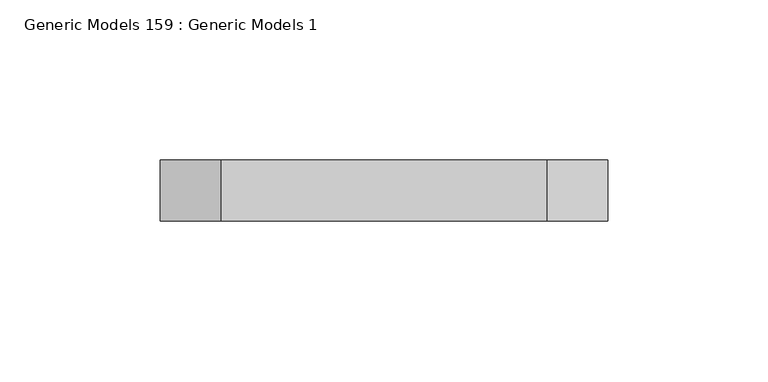
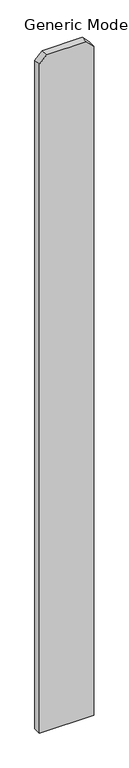
"""IFC4 building model written with IfcOpenShell, lengths in millimetres: proxy geometry, Generic Models 159 : Generic Models 1."""

import ifcopenshell
import ifcopenshell.guid

model = None  # the IFC model being written
_history = None  # IfcOwnerHistory: only IFC2X3 demands one
_inside = {}  # id of a spatial element -> (the spatial element, [elements in it])
_under = {}  # id of a project, library or spatial element -> (it, [spatial elements below it])
_declared = {}  # id of a project -> (the project, [libraries it declares])
_typed = {}  # id of a type object -> (the type object, [elements of that type])
_made_of = {}  # id of a material, layer set ... -> (it, [elements and type objects made of it])


def new_model(schema):
    """Start an empty IFC model of exactly this schema.

    Asked for "IFC4X3", IfcOpenShell would pick the latest addendum, in which some entities
    have other attributes; the version numbers below select the first issue.
    IFC2X3 requires an IfcOwnerHistory on every rooted entity: one is made here for all.
    """
    global model, _history
    if schema == "IFC4X3":
        model = ifcopenshell.file(schema_version=(4, 3, 0, 0))
    else:
        model = ifcopenshell.file(schema=schema)
    _inside.clear()
    _under.clear()
    _declared.clear()
    _typed.clear()
    _made_of.clear()
    _history = None
    if model.schema == "IFC2X3":
        org = make("IfcOrganization", Name="unknown")
        user = make(
            "IfcPersonAndOrganization",
            ThePerson=make("IfcPerson", FamilyName="unknown"),
            TheOrganization=org,
        )
        app = make(
            "IfcApplication",
            ApplicationDeveloper=org,
            Version="unknown",
            ApplicationFullName="unknown",
            ApplicationIdentifier="unknown",
        )
        _history = make(
            "IfcOwnerHistory",
            OwningUser=user,
            OwningApplication=app,
            ChangeAction="ADDED",
            CreationDate=0,
        )
    return model


def make(cls, **values):
    """One entity of the class cls with the attributes given. An attribute that is None is left unset."""
    return model.create_entity(
        cls, **{name: value for name, value in values.items() if value is not None}
    )


def rooted(cls, **values):
    """An entity with a GlobalId (a new one), such as an element, a storey or a relation."""
    return make(cls, GlobalId=ifcopenshell.guid.new(), OwnerHistory=_history, **values)


def si_unit(unit_type, name, prefix=None):
    """IfcSIUnit, for example si_unit("LENGTHUNIT", "METRE", prefix="MILLI")."""
    return make("IfcSIUnit", UnitType=unit_type, Prefix=prefix, Name=name)


def assignment(units):
    """IfcUnitAssignment: the units of a project."""
    return None if units is None else make("IfcUnitAssignment", Units=units)


def point(xyz):
    """IfcCartesianPoint."""
    return None if xyz is None else make("IfcCartesianPoint", Coordinates=xyz)


def direction(xyz):
    """IfcDirection."""
    return None if xyz is None else make("IfcDirection", DirectionRatios=xyz)


def frame(location, z_axis=None, x_axis=None):
    """IfcAxis2Placement3D, a coordinate frame: its origin and axes. An axis left out is left unset."""
    return make(
        "IfcAxis2Placement3D",
        Location=point(location),
        Axis=direction(z_axis),
        RefDirection=direction(x_axis),
    )


def origin():
    """The frame at (0, 0, 0) with its axes left unset."""
    return frame((0.0, 0.0, 0.0))


def place(relative_to, where):
    """IfcLocalPlacement: puts the frame where relative to a parent placement (None: the world)."""
    return make(
        "IfcLocalPlacement", PlacementRelTo=relative_to, RelativePlacement=where
    )


def context(
    kind, dimensions, precision=None, world=None, true_north=None, identifier=None
):
    """IfcGeometricRepresentationContext, for example the 3D "Model" context."""
    return make(
        "IfcGeometricRepresentationContext",
        ContextIdentifier=identifier,
        ContextType=kind,
        CoordinateSpaceDimension=dimensions,
        Precision=precision,
        WorldCoordinateSystem=world,
        TrueNorth=true_north,
    )


def project(units=None, contexts=None):
    """IfcProject with its units and contexts."""
    return rooted(
        "IfcProject",
        Name="project",
        RepresentationContexts=contexts,
        UnitsInContext=assignment(units),
    )


def spatial(cls, under=None, at=None, **own):
    """A site, building, storey or space (cls), placed at a placement, below another one or the project."""
    s = rooted(cls, ObjectPlacement=at, **own)
    if under is not None:
        _under.setdefault(under.id(), (under, []))[1].append(s)
    return s


def polyline(points):
    """IfcPolyline through the points."""
    return make("IfcPolyline", Points=[point(p) for p in points])


def outline(outer, holes=None, kind="AREA"):
    """IfcArbitraryClosedProfileDef: a profile drawn as a closed curve; with holes, ...WithVoids."""
    if holes is None:
        return make("IfcArbitraryClosedProfileDef", ProfileType=kind, OuterCurve=outer)
    return make(
        "IfcArbitraryProfileDefWithVoids",
        ProfileType=kind,
        OuterCurve=outer,
        InnerCurves=holes,
    )


def extrude(swept, where, along, depth):
    """IfcExtrudedAreaSolid: the profile swept, set in the frame where, extruded along a direction by depth."""
    return make(
        "IfcExtrudedAreaSolid",
        SweptArea=swept,
        Position=where,
        ExtrudedDirection=direction(along),
        Depth=depth,
    )


def shape(context_of_items, identifier, shape_type, items):
    """IfcShapeRepresentation: the items that make up one representation, for example the "Body"."""
    return make(
        "IfcShapeRepresentation",
        ContextOfItems=context_of_items,
        RepresentationIdentifier=identifier,
        RepresentationType=shape_type,
        Items=items,
    )


def source(mapping_origin, context_of_items, identifier, shape_type, items):
    """IfcRepresentationMap: a shape defined once, which mapped items show again and again."""
    return make(
        "IfcRepresentationMap",
        MappingOrigin=mapping_origin,
        MappedRepresentation=shape(context_of_items, identifier, shape_type, items),
    )


def transform(
    local_origin,
    x_axis=None,
    y_axis=None,
    z_axis=None,
    scale=None,
    scale2=None,
    scale3=None,
    uniform=True,
):
    """IfcCartesianTransformationOperator3D, or its non-uniform kind. x_axis, y_axis, z_axis: its Axis1, 2, 3."""
    if uniform:
        return make(
            "IfcCartesianTransformationOperator3D",
            Axis1=direction(x_axis),
            Axis2=direction(y_axis),
            LocalOrigin=point(local_origin),
            Scale=scale,
            Axis3=direction(z_axis),
        )
    return make(
        "IfcCartesianTransformationOperator3DnonUniform",
        Axis1=direction(x_axis),
        Axis2=direction(y_axis),
        LocalOrigin=point(local_origin),
        Scale=scale,
        Axis3=direction(z_axis),
        Scale2=scale2,
        Scale3=scale3,
    )


def mapped(mapping_source, mapping_target):
    """IfcMappedItem: shows the shape of a source again, moved by a transform."""
    return make(
        "IfcMappedItem", MappingSource=mapping_source, MappingTarget=mapping_target
    )


def made_of(thing, what):
    """Note that an element or type object is made of a material, layer set ...; save() writes the relation."""
    if what is not None:
        _made_of.setdefault(what.id(), (what, []))[1].append(thing)
    return thing


def element(
    cls,
    number,
    at=None,
    inside=None,
    cuts=None,
    type_object=None,
    material=None,
    context=None,
    identifier="Body",
    shape_type=None,
    held_by="IfcProductDefinitionShape",
    body=None,
    shapes=None,
    **own,
):
    """One element of the class cls, such as IfcWall. Its Tag is "e" and its number.

    at: its placement. inside: the storey or other place that contains it. cuts: it is an
    opening in that element (IfcRelVoidsElement). A single representation is given by context,
    identifier, shape_type and body (its items); several are given by shapes. held_by: the class
    of the entity that holds the representations. save() writes the other relations.
    """
    e = rooted(cls, Tag="e%d" % number, ObjectPlacement=at, **own)
    if body is not None:
        shapes = [shape(context, identifier, shape_type, body)]
    if shapes is not None:
        e.Representation = make(held_by, Representations=shapes)
    if inside is not None:
        _inside.setdefault(inside.id(), (inside, []))[1].append(e)
    if cuts is not None:
        rooted(
            "IfcRelVoidsElement", RelatingBuildingElement=cuts, RelatedOpeningElement=e
        )
    if type_object is not None:
        _typed.setdefault(type_object.id(), (type_object, []))[1].append(e)
    return made_of(e, material)


def aggregate(whole, parts):
    """IfcRelAggregates: a whole, such as a stair, and the parts it consists of."""
    return rooted("IfcRelAggregates", RelatingObject=whole, RelatedObjects=parts)


def save(model, path):
    """Write the relations noted so far, then the file.

    IfcRelAggregates (storeys below a building ...), IfcRelContainedInSpatialStructure (elements
    in a storey), IfcRelDefinesByType, IfcRelAssociatesMaterial and IfcRelDeclares: one each for
    every whole, place, type object, material and project.
    """
    for whole, parts in _under.values():
        aggregate(whole, parts)
    for where, things in _inside.values():
        rooted(
            "IfcRelContainedInSpatialStructure",
            RelatedElements=things,
            RelatingStructure=where,
        )
    for kind, things in _typed.values():
        rooted("IfcRelDefinesByType", RelatedObjects=things, RelatingType=kind)
    for what, things in _made_of.values():
        rooted("IfcRelAssociatesMaterial", RelatedObjects=things, RelatingMaterial=what)
    for by, libraries in _declared.values():
        rooted("IfcRelDeclares", RelatingContext=by, RelatedDefinitions=libraries)
    model.write(path)


def generic_models_159_generic_models_1_27e70c3d(model_context):
    return source(origin(), model_context, "Body", "SweptSolid", [
        extrude(outline(polyline([(76.2, 54227.4125), (1885.95, 54227.4125), (1905.0, 54208.3625), (1905.0, 54106.7625), (1885.95, 54087.7125), (76.2, 54087.7125), (76.2, 54227.4125)])), frame((0.0, 547.6875, 0.0), z_axis=(0.0, 1.0, 0.0), x_axis=(0.0, 0.0, 1.0)), (0.0, 0.0, 1.0), 19.05),
    ])


if __name__ == "__main__":
    model = new_model("IFC4")
    model_context = context("Model", 3, world=origin())
    ifc_project = project(units=[si_unit("LENGTHUNIT", "METRE", prefix="MILLI")], contexts=[model_context])
    site = spatial("IfcSite", under=ifc_project)
    building = spatial("IfcBuilding", under=site)
    placement = place(None, origin())
    generic_models_159_generic_models_1_shape = generic_models_159_generic_models_1_27e70c3d(model_context)
    element("IfcBuildingElementProxy", 1, Name="Generic Models 159 : Generic Models 1", ObjectType="Generic Models 159 : Generic Models 1", at=placement, inside=building, context=model_context, shape_type="MappedRepresentation", body=[
        mapped(generic_models_159_generic_models_1_shape, transform((0.0, 0.0, 0.0), x_axis=(1.0, 0.0, 0.0), y_axis=(0.0, 1.0, 0.0), z_axis=(0.0, 0.0, 1.0))),
    ])
    save(model, "model.ifc")

# Revit data of these elements
# Element 1 (IfcBuildingElementProxy, "Generic Models 159 : Generic Models 1")
#   Materials on its faces: "VERTICAL 1X6 CEDAR PLANKS W/ CLEAR WOOD SEALER"
# Materials
#   "VERTICAL 1X6 CEDAR PLANKS W/ CLEAR WOOD SEALER": class "Wood", colour RGB 234 198 147, transparency 0, Description = "Pinus Echinata", Cost = 0
